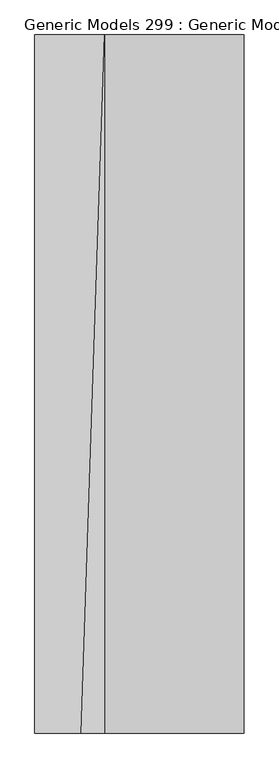
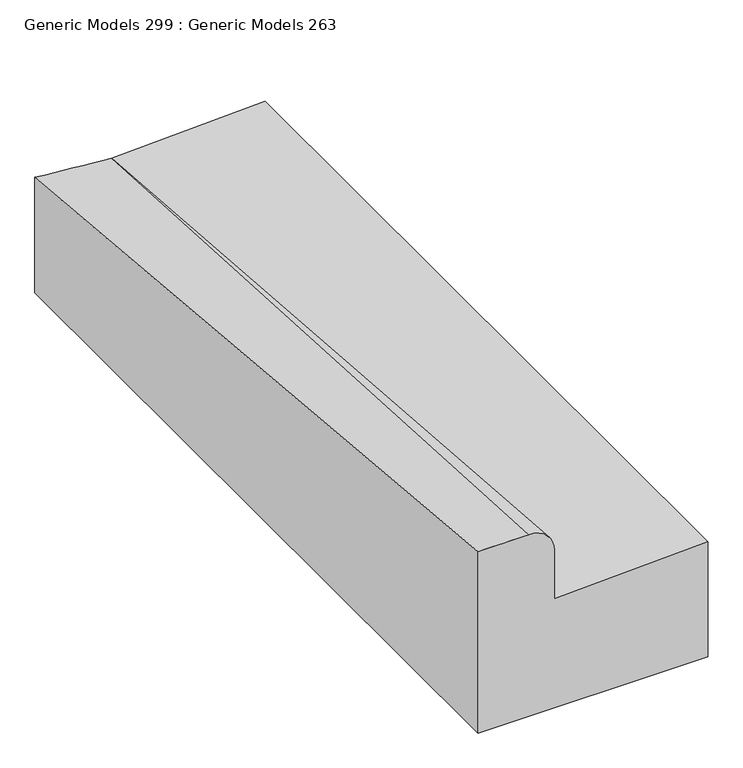
"""IFC4 building model written with IfcOpenShell, lengths in millimetres: proxy geometry, Generic Models 299 : Generic Models 263."""

from ifc_helpers import new_model, si_unit, frame, origin, place, context, project, spatial, circle_curve, source, transform, mapped, element, save
from ifc_brep_helpers import plane_surface, spline_surface, advanced_brep


def generic_models_299_generic_models_263_ab59c33a(model_context):
    return source(origin(), model_context, "Body", "AdvancedBrep", [
        advanced_brep(
        [(91579.9797726, -6732.6272578, -139.1379392), (91732.3797726, -6732.6272578, -152.4), (92037.1797726, -6732.6272578, -139.7), (92037.1797726, -6732.6272578, -381.0), (91579.9797726, -6732.6272578, -381.0), (91579.9797726, -8256.6272578, 0.0), (91579.9797726, -8256.6272578, -381.0), (92037.1797726, -8256.6272578, -381.0), (92037.1797726, -8256.6272578, -139.7), (91732.3797726, -8256.6272578, -152.4), (91732.3797726, -8256.6272578, -50.8), (91681.5797726, -8256.6272578, 0.0)],
        [
            (0, 1),
            (1, 2),
            (2, 3),
            (3, 4),
            (4, 0),
            (5, 6),
            (6, 7),
            (7, 8),
            (8, 9),
            (9, 10),
            (10, 11, circle_curve(frame((91681.5797726, -8256.6272578, -50.8), z_axis=(0.0, -1.0, 0.0), x_axis=(1.0, 0.0, 0.0)), 50.8)),
            (11, 5),
            (5, 0),
            (4, 6),
            (3, 7),
            (2, 8),
            (9, 1),
            (1, 10),
            (1, 11),
        ],
        [
            plane_surface(frame((91793.3397726, -6732.6272578, -238.6475878), z_axis=(0.0, 1.0, 0.0), x_axis=(0.0, 0.0, 1.0))),
            plane_surface(frame((91768.6654869, -8256.6272578, -157.8428571), z_axis=(0.0, -1.0, 0.0), x_axis=(0.0, 0.0, 1.0))),
            plane_surface(frame((91579.9797726, -8256.6272578, -190.5), z_axis=(-1.0, 0.0, 0.0), x_axis=(0.0, 0.0, 1.0))),
            plane_surface(frame((91808.5797726, -8256.6272578, -381.0), z_axis=(0.0, 0.0, -1.0), x_axis=(-1.0, 0.0, 0.0))),
            plane_surface(frame((92037.1797726, -8256.6272578, -260.35), z_axis=(1.0, 0.0, 0.0), x_axis=(0.0, 0.0, -1.0))),
            plane_surface(frame((91732.3797726, -8256.6272578, -101.6), z_axis=(1.0, 0.0, 0.0), x_axis=(0.0, 0.0, -1.0))),
            spline_surface(2, 1, [[(91681.5797726, -8256.6272578, 0.0), (91732.3797726, -6732.6272578, -152.4)], [(91732.3797726, -8256.6272578, -2.9132252166164108e-12), (91732.3797726, -6732.6272578, -152.4)], [(91732.3797726, -8256.6272578, -50.8), (91732.3797726, -6732.6272578, -152.4)]], [3, 3], [2, 2], [0.0, 1.0], [0.0, 1.0], weights=[[1.0, 1.0], [0.7071067811865678, 0.7071067811865678], [1.0, 1.0]]),
            spline_surface(1, 1, [[(91579.9797726, -8256.6272578, 0.0), (91579.9797726, -6732.6272578, -139.1379392)], [(91681.5797726, -8256.6272578, 0.0), (91732.3797726, -6732.6272578, -152.4)]], [2, 2], [2, 2], [0.0, 1.0], [0.0, 1.0]),
            plane_surface(frame((91884.7797726, -8256.6272578, -146.05), z_axis=(-0.04163054471218606, 0.0, 0.9991330730923518), x_axis=(0.9991330730923518, 0.0, 0.04163054471218606))),
        ],
        [
            (0, [[1, 2, 3, 4, 5]]),
            (1, [[6, 7, 8, 9, 10, 11, 12]]),
            (2, [[-6, 13, -5, 14]]),
            (3, [[-7, -14, -4, 15]]),
            (4, [[-8, -15, -3, 16]]),
            (5, [[-10, 17, 18]]),
            (6, [[-11, -18, 19]]),
            (7, [[-12, -19, -1, -13]]),
            (8, [[-9, -16, -2, -17]]),
        ],
    ),
    ])


if __name__ == "__main__":
    model = new_model("IFC4")
    model_context = context("Model", 3, world=origin())
    ifc_project = project(units=[si_unit("LENGTHUNIT", "METRE", prefix="MILLI")], contexts=[model_context])
    site = spatial("IfcSite", under=ifc_project)
    building = spatial("IfcBuilding", under=site)
    placement = place(None, origin())
    generic_models_299_generic_models_263_shape = generic_models_299_generic_models_263_ab59c33a(model_context)
    element("IfcBuildingElementProxy", 1, Name="Generic Models 299 : Generic Models 263", ObjectType="Generic Models 299 : Generic Models 263", at=placement, inside=building, context=model_context, shape_type="MappedRepresentation", body=[
        mapped(generic_models_299_generic_models_263_shape, transform((0.0, 0.0, 0.0), x_axis=(1.0, 0.0, 0.0), y_axis=(0.0, 1.0, 0.0), z_axis=(0.0, 0.0, 1.0))),
    ])
    save(model, "model.ifc")

# Revit data of these elements
# Element 1 (IfcBuildingElementProxy, "Generic Models 299 : Generic Models 263")
#   Materials on its faces: "CONCRETE CURB"
# Materials
#   "CONCRETE CURB": class "Concrete", colour RGB 191 191 191, transparency 0, Description = "Cast-in-place concrete", Cost = 0
